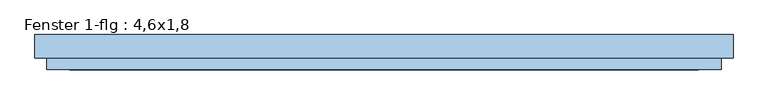
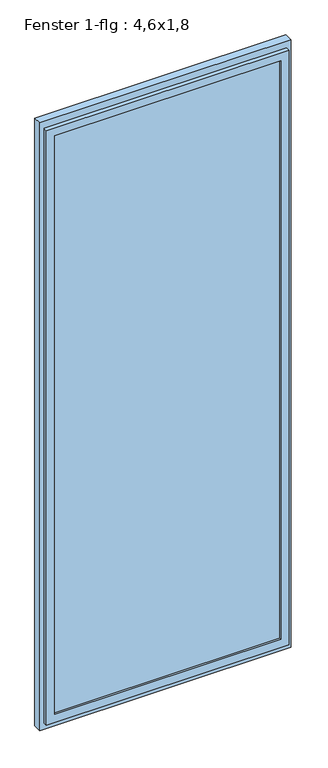
"""IFC4 building model written with IfcOpenShell, lengths in millimetres: window geometry, Fenster 1-flg : 4,6x1,8."""

from ifc_helpers import new_model, si_unit, frame, origin, place, context, project, spatial, polyline, outline, extrude, faceted_brep, source, transform, mapped, element, save


def fenster_1_flg_4_6x1_8_3e6bb3fe(model_context):
    return source(origin(), model_context, "Body", "SolidModel", [
        extrude(outline(polyline([(5600.0, 900.0), (5600.0, -900.0), (1000.0, -900.0), (1000.0, 900.0), (5600.0, 900.0)]), holes=[polyline([(5520.0, 840.0), (1080.0, 840.0), (1080.0, -840.0), (5520.0, -840.0), (5520.0, 840.0)])]), frame((0.0, 20.0, 0.0), z_axis=(0.0, 1.0, 0.0), x_axis=(0.0, 0.0, 1.0)), (0.0, 0.0, 1.0), 60.0),
        faceted_brep([(870.0, 20.0, 5550.0), (870.0, -10.0, 5550.0), (870.0, -10.0, 1050.0), (870.0, 20.0, 1050.0), (-870.0, -10.0, 5550.0), (-870.0, -10.0, 1050.0), (810.0, -10.0, 1110.0), (-810.0, -10.0, 1110.0), (-810.0, -10.0, 5490.0), (810.0, -10.0, 5490.0), (-870.0, 20.0, 1050.0), (-870.0, 20.0, 5550.0), (840.0, 20.0, 5520.0), (-840.0, 20.0, 5520.0), (-840.0, 20.0, 1080.0), (840.0, 20.0, 1080.0), (840.0, 50.0, 5520.0), (840.0, 50.0, 1080.0), (-840.0, 50.0, 1080.0), (-840.0, 50.0, 5520.0), (810.0, 50.0, 5490.0), (-810.0, 50.0, 5490.0), (-810.0, 50.0, 1110.0), (810.0, 50.0, 1110.0)], [[[0, 1, 2, 3]], [[1, 4, 5, 2], [6, 7, 8, 9]], [[3, 2, 5, 10]], [[3, 10, 11, 0], [12, 13, 14, 15]], [[16, 12, 15, 17]], [[17, 15, 14, 18]], [[17, 18, 19, 16], [20, 21, 22, 23]], [[9, 20, 23, 6]], [[6, 23, 22, 7]], [[10, 5, 4, 11]], [[18, 14, 13, 19]], [[7, 22, 21, 8]], [[11, 4, 1, 0]], [[19, 13, 12, 16]], [[8, 21, 20, 9]]]),
        extrude(outline(polyline([(810.0, 5.0), (-810.0, 5.0), (-810.0, 35.0), (810.0, 35.0), (810.0, 5.0)])), frame((0.0, 0.0, 1110.0), z_axis=(0.0, 0.0, 1.0), x_axis=(1.0, 0.0, 0.0)), (0.0, 0.0, 1.0), 4380.0),
    ])


if __name__ == "__main__":
    model = new_model("IFC4")
    model_context = context("Model", 3, world=origin())
    ifc_project = project(units=[si_unit("LENGTHUNIT", "METRE", prefix="MILLI")], contexts=[model_context])
    site = spatial("IfcSite", under=ifc_project)
    building = spatial("IfcBuilding", under=site)
    placement = place(None, origin())
    fenster_1_flg_4_6x1_8_shape = fenster_1_flg_4_6x1_8_3e6bb3fe(model_context)
    element("IfcWindow", 1, ObjectType="Fenster 1-flg : 4,6x1,8", at=placement, inside=building, context=model_context, shape_type="MappedRepresentation", body=[
        mapped(fenster_1_flg_4_6x1_8_shape, transform((0.0, 0.0, 0.0), x_axis=(1.0, 0.0, 0.0), y_axis=(0.0, 1.0, 0.0), z_axis=(0.0, 0.0, 1.0))),
    ])
    save(model, "model.ifc")

# Revit data of these elements
# Type "Fenster 1-flg : 4,6x1,8"
#   Type Mark = "68"
#   Operation = "SinglePanel"
#   Keynote = "16.05.01"
#   Visual Light Transmittance = 0.9
#   Solar Heat Gain Coefficient = 0.86
#   Rough Width = 1.800 m
#   Rough Height = 4.600 m
#   Heat Transfer Coefficient (U) = 5.5617 W/(m²·K)
#   Rahmentiefe = 0.060 m
#   Rahmenhöhe - unten = 0.080 m
#   Rahmenhöhe - oben = 0.080 m
#   Rahmenbreite = 0.060 m
#   Height = 4.600 m
#   Tiefe Flügel = 0.060 m
#   Flügelbreite = 0.060 m
#   Einbautiefe (von außen) [instance default] = 0.100 m
#   Width = 1.800 m
#   Klappflügel [instance default] = no
#   Kippflügel [instance default] = yes
#   Öffnungsrichtung in Draufsicht anzeigen [instance default] = no
#   Drehflügel 1 [instance default] = yes
#   Rahmen 1 [instance default] = none
#   Glas [instance default] = none
#   Flügel [instance default] = none
#   Fensterbank Innenseite [instance default] = none
#   Fensterbank Außenseite [instance default] = none
#   Construction Type Id = ""
#   Wall Closure = (empty or 0)
#   Analytic Construction = (empty or 0)
# Element 1 (IfcWindow, "Fenster 1-flg : 4,6x1,8")
#   Einbautiefe (von außen) = 0.230 m
#   Materials on its faces: "Kunststoff - Weiß", "Glas"
# Materials
#   "Kunststoff - Weiß": class "Kunststoff", colour RGB 249 249 249, transparency 0, Cost = 0
#   "Glas": class "Glas", colour RGB 0 0 255, transparency 0.75, Comments = "Render-Darstellung nicht aktualisiert ", Cost = 0
